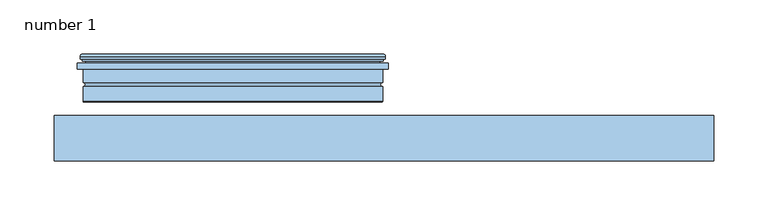
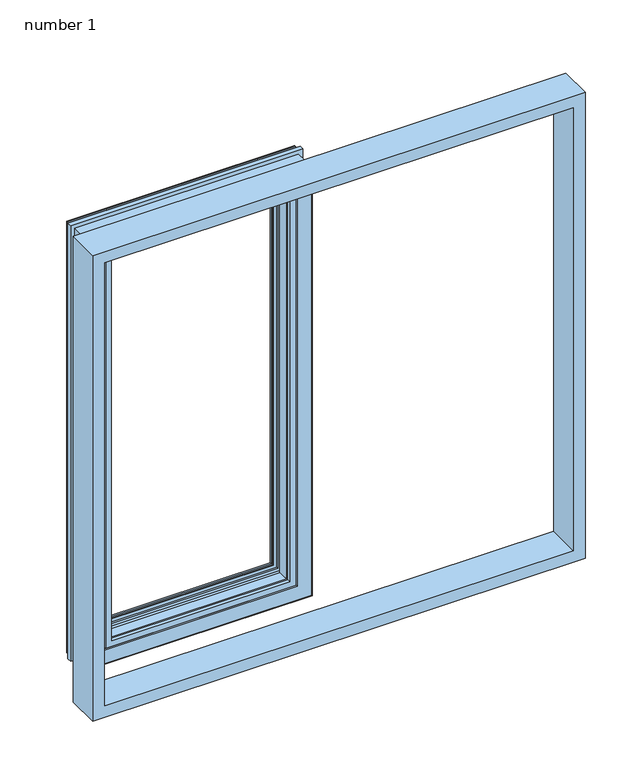
"""IFC4 building model written with IfcOpenShell, lengths in millimetres: window geometry, Window-Exterior-Sierra-Horizontal_Sliding_XO-36inch_Width-Standard : number 1."""

from ifc_helpers import new_model, si_unit, frame, origin, place, context, project, spatial, polyline, ellipse_curve, outline, extrude, source, transform, mapped, element, save
from ifc_brep_helpers import plane_surface, cylinder_surface, revolved_surface, advanced_brep


def number_1_632643b2(model_context):
    return source(origin(), model_context, "Body", "SolidModel", [
        advanced_brep(
        [(-250.12015, 35.099625, 967.49235), (-250.12015, 33.9637671, 967.49235), (-29.27985, 33.9637671, 967.49235), (-29.27985, 35.099625, 967.49235), (-248.2833265, 37.5426644, 969.3291735), (-248.0937762, 35.099625, 969.5187238), (-31.3062238, 35.099625, 969.5187238), (-31.1166735, 37.5426644, 969.3291735), (-256.08915, 40.078025, 961.52335), (-23.31085, 40.078025, 961.52335), (-256.08915, 42.465625, 961.52335), (-23.31085, 42.465625, 961.52335), (-280.77795, 40.078025, 936.83455), (-278.39035, 42.465625, 939.22215), (-1.00965, 42.465625, 939.22215), (1.37795, 40.078025, 936.83455), (-280.77795, 37.512625, 936.83455), (1.37795, 37.512625, 936.83455), (-278.74595, 35.836225, 938.86655), (-278.74595, 37.512625, 938.86655), (-0.65405, 37.512625, 938.86655), (-0.65405, 35.836225, 938.86655), (-275.44395, 33.931225, 942.16855), (-275.44395, 35.836225, 942.16855), (-3.95605, 35.836225, 942.16855), (-3.95605, 33.931225, 942.16855), (-283.36875, 28.317825, 934.24375), (-283.36875, 33.931225, 934.24375), (3.96875, 33.931225, 934.24375), (3.96875, 28.317825, 934.24375), (-278.06015, 16.125825, 939.55235), (-278.06015, 28.317825, 939.55235), (-1.33985, 28.317825, 939.55235), (-1.33985, 16.125825, 939.55235), (-278.06015, 12.163425, 939.55235), (-1.33985, 12.163425, 939.55235), (-278.06015, -1.171575, 939.55235), (-1.33985, -1.171575, 939.55235), (-277.24735, -1.984375, 940.36515), (-2.15265, -1.984375, 940.36515), (-258.95935, -0.103857, 958.65315), (-258.95935, -1.984375, 958.65315), (-20.44065, -1.984375, 958.65315), (-20.44065, -0.103857, 958.65315), (-257.3584612, -1.704057, 960.2540388), (-257.3584612, -0.103857, 960.2540388), (-22.0415388, -0.103857, 960.2540388), (-22.0415388, -1.704057, 960.2540388), (-249.8146612, 2.0638625, 967.7978388), (-249.8146612, -1.704057, 967.7978388), (-29.5853388, -1.704057, 967.7978388), (-29.5853388, 2.0638625, 967.7978388), (-246.6396612, 13.891543, 970.9728388), (-247.6523112, 2.0638625, 969.9601888), (-31.7476888, 2.0638625, 969.9601888), (-32.7603388, 13.891543, 970.9728388), (-258.95935, 11.5032541, 958.65315), (-256.5710612, 13.891543, 961.0414388), (-22.8289388, 13.891543, 961.0414388), (-20.44065, 11.5032541, 958.65315), (-258.95935, 32.940625, 958.65315), (-20.44065, 32.940625, 958.65315), (-254.3555891, 33.9637671, 963.2569109), (-255.3787312, 32.940625, 962.2337688), (-24.0212688, 32.940625, 962.2337688), (-25.0444109, 33.9637671, 963.2569109), (-29.27985, 33.9637671, 1470.90765), (-29.27985, 35.099625, 1470.90765), (-31.3062238, 35.099625, 1468.8812762), (-31.1166735, 37.5426644, 1469.0708265), (-23.31085, 40.078025, 1476.87665), (-23.31085, 42.465625, 1476.87665), (-1.00965, 42.465625, 1499.17785), (1.37795, 40.078025, 1501.56545), (1.37795, 37.512625, 1501.56545), (-0.65405, 37.512625, 1499.53345), (-0.65405, 35.836225, 1499.53345), (-3.95605, 35.836225, 1496.23145), (-3.95605, 33.931225, 1496.23145), (3.96875, 33.931225, 1504.15625), (3.96875, 28.317825, 1504.15625), (-1.33985, 28.317825, 1498.84765), (-1.33985, 16.125825, 1498.84765), (-1.33985, 12.163425, 1498.84765), (-1.33985, -1.171575, 1498.84765), (-2.15265, -1.984375, 1498.03485), (-20.44065, -1.984375, 1479.74685), (-20.44065, -0.103857, 1479.74685), (-22.0415388, -0.103857, 1478.1459612), (-22.0415388, -1.704057, 1478.1459612), (-29.5853388, -1.704057, 1470.6021612), (-29.5853388, 2.0638625, 1470.6021612), (-31.7476888, 2.0638625, 1468.4398112), (-32.7603388, 13.891543, 1467.4271612), (-22.8289388, 13.891543, 1477.3585612), (-20.44065, 11.5032541, 1479.74685), (-20.44065, 32.940625, 1479.74685), (-24.0212688, 32.940625, 1476.1662312), (-25.0444109, 33.9637671, 1475.1430891), (-250.12015, 33.9637671, 1470.90765), (-250.12015, 35.099625, 1470.90765), (-248.0937762, 35.099625, 1468.8812762), (-248.2833265, 37.5426644, 1469.0708265), (-256.08915, 40.078025, 1476.87665), (-256.08915, 42.465625, 1476.87665), (-278.39035, 42.465625, 1499.17785), (-280.77795, 40.078025, 1501.56545), (-280.77795, 37.512625, 1501.56545), (-278.74595, 37.512625, 1499.53345), (-278.74595, 35.836225, 1499.53345), (-275.44395, 35.836225, 1496.23145), (-275.44395, 33.931225, 1496.23145), (-283.36875, 33.931225, 1504.15625), (-283.36875, 28.317825, 1504.15625), (-278.06015, 28.317825, 1498.84765), (-278.06015, 16.125825, 1498.84765), (-278.06015, 12.163425, 1498.84765), (-278.06015, -1.171575, 1498.84765), (-277.24735, -1.984375, 1498.03485), (-258.95935, -1.984375, 1479.74685), (-258.95935, -0.103857, 1479.74685), (-257.3584612, -0.103857, 1478.1459612), (-257.3584612, -1.704057, 1478.1459612), (-249.8146612, -1.704057, 1470.6021612), (-249.8146612, 2.0638625, 1470.6021612), (-247.6523112, 2.0638625, 1468.4398112), (-246.6396612, 13.891543, 1467.4271612), (-256.5710612, 13.891543, 1477.3585612), (-258.95935, 11.5032541, 1479.74685), (-258.95935, 32.940625, 1479.74685), (-255.3787312, 32.940625, 1476.1662312), (-254.3555891, 33.9637671, 1475.1430891)],
        [
            (0, 1),
            (1, 2),
            (2, 3),
            (3, 0),
            (4, 5),
            (5, 6),
            (6, 7),
            (7, 4),
            (8, 4),
            (7, 9),
            (9, 8),
            (10, 8),
            (9, 11),
            (11, 10),
            (12, 13, ellipse_curve(frame((-278.39035, 40.078025, 939.22215), z_axis=(0.7071067811865475, 0.0, -0.7071067811865475), x_axis=(-0.7071067811865476, 0.0, -0.7071067811865474)), 3.3765763, 2.3876)),
            (13, 14),
            (14, 15, ellipse_curve(frame((-1.00965, 40.078025, 939.22215), z_axis=(-0.7071067811865475, 0.0, -0.7071067811865475), x_axis=(-0.7071067811865476, 0.0, 0.7071067811865474)), 3.3765763, 2.3876)),
            (15, 12),
            (16, 12),
            (15, 17),
            (17, 16),
            (18, 19),
            (19, 20),
            (20, 21),
            (21, 18),
            (22, 23),
            (23, 24),
            (24, 25),
            (25, 22),
            (26, 27),
            (27, 28),
            (28, 29),
            (29, 26),
            (30, 31),
            (31, 32),
            (32, 33),
            (33, 30),
            (34, 30, ellipse_curve(frame((-278.06015, 14.144625, 939.55235), z_axis=(-0.7071067811865475, 0.0, 0.7071067811865475), x_axis=(0.7071067811865476, 0.0, 0.7071067811865474)), 2.8018399, 1.9812)),
            (33, 35, ellipse_curve(frame((-1.33985, 14.144625, 939.55235), z_axis=(0.7071067811865475, 0.0, 0.7071067811865475), x_axis=(0.7071067811865476, 0.0, -0.7071067811865474)), 2.8018399, 1.9812)),
            (35, 34),
            (36, 34),
            (35, 37),
            (37, 36),
            (38, 36, ellipse_curve(frame((-277.24735, -1.171575, 940.36515), z_axis=(0.7071067811865475, 0.0, -0.7071067811865475), x_axis=(-0.7071067811865476, 0.0, -0.7071067811865474)), 1.1494728, 0.8128)),
            (37, 39, ellipse_curve(frame((-2.15265, -1.171575, 940.36515), z_axis=(-0.7071067811865475, 0.0, -0.7071067811865475), x_axis=(-0.7071067811865476, 0.0, 0.7071067811865474)), 1.1494728, 0.8128)),
            (39, 38),
            (40, 41),
            (41, 42),
            (42, 43),
            (43, 40),
            (44, 45),
            (45, 46),
            (46, 47),
            (47, 44),
            (48, 49),
            (49, 50),
            (50, 51),
            (51, 48),
            (52, 53),
            (53, 54),
            (54, 55),
            (55, 52),
            (56, 57),
            (57, 58),
            (58, 59),
            (59, 56),
            (60, 56),
            (59, 61),
            (61, 60),
            (62, 63),
            (63, 64),
            (64, 65),
            (65, 62),
            (2, 66),
            (66, 67),
            (67, 3),
            (6, 68),
            (68, 69),
            (69, 7),
            (69, 70),
            (70, 9),
            (70, 71),
            (71, 11),
            (14, 72),
            (72, 73, ellipse_curve(frame((-1.00965, 40.078025, 1499.17785), z_axis=(0.7071067811865475, 0.0, -0.7071067811865475), x_axis=(-0.7071067811865474, 0.0, -0.7071067811865476)), 3.3765763, 2.3876)),
            (73, 15),
            (73, 74),
            (74, 17),
            (20, 75),
            (75, 76),
            (76, 21),
            (24, 77),
            (77, 78),
            (78, 25),
            (28, 79),
            (79, 80),
            (80, 29),
            (32, 81),
            (81, 82),
            (82, 33),
            (82, 83, ellipse_curve(frame((-1.33985, 14.144625, 1498.84765), z_axis=(-0.7071067811865475, 0.0, 0.7071067811865475), x_axis=(0.7071067811865474, 0.0, 0.7071067811865476)), 2.8018399, 1.9812)),
            (83, 35),
            (83, 84),
            (84, 37),
            (84, 85, ellipse_curve(frame((-2.15265, -1.171575, 1498.03485), z_axis=(0.7071067811865475, 0.0, -0.7071067811865475), x_axis=(-0.7071067811865474, 0.0, -0.7071067811865476)), 1.1494728, 0.8128)),
            (85, 39),
            (42, 86),
            (86, 87),
            (87, 43),
            (46, 88),
            (88, 89),
            (89, 47),
            (50, 90),
            (90, 91),
            (91, 51),
            (54, 92),
            (92, 93),
            (93, 55),
            (58, 94),
            (94, 95),
            (95, 59),
            (95, 96),
            (96, 61),
            (64, 97),
            (97, 98),
            (98, 65),
            (66, 99),
            (99, 100),
            (100, 67),
            (68, 101),
            (101, 102),
            (102, 69),
            (102, 103),
            (103, 70),
            (103, 104),
            (104, 71),
            (72, 105),
            (105, 106, ellipse_curve(frame((-278.39035, 40.078025, 1499.17785), z_axis=(0.7071067811865475, 0.0, 0.7071067811865475), x_axis=(0.7071067811865476, 0.0, -0.7071067811865474)), 3.3765763, 2.3876)),
            (106, 73),
            (106, 107),
            (107, 74),
            (75, 108),
            (108, 109),
            (109, 76),
            (77, 110),
            (110, 111),
            (111, 78),
            (79, 112),
            (112, 113),
            (113, 80),
            (81, 114),
            (114, 115),
            (115, 82),
            (115, 116, ellipse_curve(frame((-278.06015, 14.144625, 1498.84765), z_axis=(-0.7071067811865475, 0.0, -0.7071067811865475), x_axis=(-0.7071067811865476, 0.0, 0.7071067811865474)), 2.8018399, 1.9812)),
            (116, 83),
            (116, 117),
            (117, 84),
            (117, 118, ellipse_curve(frame((-277.24735, -1.171575, 1498.03485), z_axis=(0.7071067811865475, 0.0, 0.7071067811865475), x_axis=(0.7071067811865476, 0.0, -0.7071067811865474)), 1.1494728, 0.8128)),
            (118, 85),
            (86, 119),
            (119, 120),
            (120, 87),
            (88, 121),
            (121, 122),
            (122, 89),
            (90, 123),
            (123, 124),
            (124, 91),
            (92, 125),
            (125, 126),
            (126, 93),
            (94, 127),
            (127, 128),
            (128, 95),
            (128, 129),
            (129, 96),
            (97, 130),
            (130, 131),
            (131, 98),
            (131, 62),
            (1, 99),
            (0, 100),
            (5, 101),
            (4, 102),
            (8, 103),
            (10, 104),
            (13, 105),
            (12, 106),
            (16, 107),
            (19, 108),
            (18, 109),
            (23, 110),
            (22, 111),
            (27, 112),
            (26, 113),
            (31, 114),
            (30, 115),
            (34, 116),
            (36, 117),
            (38, 118),
            (41, 119),
            (40, 120),
            (45, 121),
            (44, 122),
            (49, 123),
            (48, 124),
            (53, 125),
            (52, 126),
            (57, 127),
            (56, 128),
            (60, 129),
            (63, 130),
        ],
        [
            plane_surface(frame((-250.12015, 33.9637671, 967.49235), z_axis=(0.0, 0.0, 1.0), x_axis=(1.0, 0.0, 0.0))),
            plane_surface(frame((-248.0937762, 35.099625, 969.5187238), z_axis=(0.0, 0.07735544009934271, 0.9970035786731345), x_axis=(1.0, 0.0, 0.0))),
            plane_surface(frame((-248.2833265, 37.5426644, 969.3291735), z_axis=(0.0, 0.9510889261909004, 0.3089172291683326), x_axis=(1.0, 0.0, 0.0))),
            plane_surface(frame((-256.08915, 40.078025, 961.52335), z_axis=(0.0, 0.0, 1.0), x_axis=(1.0, 0.0, 0.0))),
            cylinder_surface(frame((-283.36875, 40.078025, 939.22215), z_axis=(-1.0, 0.0, 0.0), x_axis=(0.0, -1.0, 0.0)), 2.3876),
            plane_surface(frame((-280.77795, 40.078025, 936.83455), z_axis=(0.0, 0.0, -1.0), x_axis=(1.0, 0.0, 0.0))),
            plane_surface(frame((-278.74595, 37.512625, 938.86655), z_axis=(0.0, 0.0, -1.0), x_axis=(1.0, 0.0, 0.0))),
            plane_surface(frame((-275.44395, 35.836225, 942.16855), z_axis=(0.0, 0.0, -1.0), x_axis=(1.0, 0.0, 0.0))),
            plane_surface(frame((-283.36875, 33.931225, 934.24375), z_axis=(0.0, 0.0, -1.0), x_axis=(1.0, 0.0, 0.0))),
            plane_surface(frame((-278.06015, 28.317825, 939.55235), z_axis=(0.0, 0.0, -1.0), x_axis=(1.0, 0.0, 0.0))),
            revolved_surface(polyline([(0.6413499930890225, 12.163425, 939.55235), (-280.04134999308906, 12.163425, 939.55235)]), (-283.36875, 14.144625, 939.55235), (1.0, 0.0, 0.0)),
            plane_surface(frame((-278.06015, 12.163425, 939.55235), z_axis=(0.0, 0.0, -1.0), x_axis=(1.0, 0.0, 0.0))),
            cylinder_surface(frame((-283.36875, -1.171575, 940.36515), z_axis=(-1.0, 0.0, 0.0), x_axis=(0.0, -1.0, 0.0)), 0.8128),
            plane_surface(frame((-258.95935, -1.984375, 958.65315), z_axis=(0.0, 0.0, 1.0), x_axis=(1.0, 0.0, 0.0))),
            plane_surface(frame((-257.3584612, -0.103857, 960.2540388), z_axis=(0.0, 0.0, -1.0), x_axis=(1.0, 0.0, 0.0))),
            plane_surface(frame((-249.8146612, -1.704057, 967.7978388), z_axis=(0.0, 0.0, 1.0), x_axis=(1.0, 0.0, 0.0))),
            plane_surface(frame((-247.6523112, 2.0638625, 969.9601888), z_axis=(0.0, -0.08530487454184647, 0.996354895797376), x_axis=(1.0, 0.0, 0.0))),
            plane_surface(frame((-256.5710612, 13.891543, 961.0414388), z_axis=(0.0, 0.7071067811865713, -0.7071067811865238), x_axis=(1.0, 0.0, 0.0))),
            plane_surface(frame((-258.95935, 11.5032541, 958.65315), z_axis=(0.0, 0.0, 1.0), x_axis=(1.0, 0.0, 0.0))),
            plane_surface(frame((-255.3787312, 32.940625, 962.2337688), z_axis=(0.0, -0.7071067811861558, 0.7071067811869393), x_axis=(1.0, 0.0, 0.0))),
            plane_surface(frame((-29.27985, 33.9637671, 967.49235), z_axis=(-1.0, 0.0, 0.0), x_axis=(0.0, 0.0, 1.0))),
            plane_surface(frame((-31.3062238, 35.099625, 969.5187238), z_axis=(-0.9970035786731345, 0.07735544009934266, 0.0), x_axis=(0.0, 0.0, 1.0))),
            plane_surface(frame((-31.1166735, 37.5426644, 969.3291735), z_axis=(-0.30891722916833264, 0.9510889261909004, 0.0), x_axis=(0.0, 0.0, 1.0))),
            plane_surface(frame((-23.31085, 40.078025, 961.52335), z_axis=(-1.0, 0.0, 0.0), x_axis=(0.0, 0.0, 1.0))),
            cylinder_surface(frame((-1.00965, 40.078025, 934.24375), z_axis=(0.0, 0.0, -1.0), x_axis=(0.0, -1.0, 0.0)), 2.3876),
            plane_surface(frame((1.37795, 40.078025, 936.83455), z_axis=(1.0, 0.0, 0.0), x_axis=(0.0, 0.0, 1.0))),
            plane_surface(frame((-0.65405, 37.512625, 938.86655), z_axis=(1.0, 0.0, 0.0), x_axis=(0.0, 0.0, 1.0))),
            plane_surface(frame((-3.95605, 35.836225, 942.16855), z_axis=(1.0, 0.0, 0.0), x_axis=(0.0, 0.0, 1.0))),
            plane_surface(frame((3.96875, 33.931225, 934.24375), z_axis=(1.0, 0.0, 0.0), x_axis=(0.0, 0.0, 1.0))),
            plane_surface(frame((-1.33985, 28.317825, 939.55235), z_axis=(1.0, 0.0, 0.0), x_axis=(0.0, 0.0, 1.0))),
            revolved_surface(polyline([(-1.33985, 12.163425, 1500.828849993089), (-1.33985, 12.163425, 937.571150006911)]), (-1.33985, 14.144625, 934.24375), (0.0, 0.0, 1.0)),
            plane_surface(frame((-1.33985, 12.163425, 939.55235), z_axis=(1.0, 0.0, 0.0), x_axis=(0.0, 0.0, 1.0))),
            cylinder_surface(frame((-2.15265, -1.171575, 934.24375), z_axis=(0.0, 0.0, -1.0), x_axis=(0.0, -1.0, 0.0)), 0.8128),
            plane_surface(frame((-20.44065, -1.984375, 958.65315), z_axis=(-1.0, 0.0, 0.0), x_axis=(0.0, 0.0, 1.0))),
            plane_surface(frame((-22.0415388, -0.103857, 960.2540388), z_axis=(1.0, 0.0, 0.0), x_axis=(0.0, 0.0, 1.0))),
            plane_surface(frame((-29.5853388, -1.704057, 967.7978388), z_axis=(-1.0, 0.0, 0.0), x_axis=(0.0, 0.0, 1.0))),
            plane_surface(frame((-31.7476888, 2.0638625, 969.9601888), z_axis=(-0.996354895797376, -0.08530487454184653, 0.0), x_axis=(0.0, 0.0, 1.0))),
            plane_surface(frame((-22.8289388, 13.891543, 961.0414388), z_axis=(0.7071067811865238, 0.7071067811865713, 0.0), x_axis=(0.0, 0.0, 1.0))),
            plane_surface(frame((-20.44065, 11.5032541, 958.65315), z_axis=(-1.0, 0.0, 0.0), x_axis=(0.0, 0.0, 1.0))),
            plane_surface(frame((-24.0212688, 32.940625, 962.2337688), z_axis=(-0.7071067811869393, -0.7071067811861558, 0.0), x_axis=(0.0, 0.0, 1.0))),
            plane_surface(frame((-29.27985, 33.9637671, 1470.90765), z_axis=(0.0, 0.0, -1.0), x_axis=(-1.0, 0.0, 0.0))),
            plane_surface(frame((-31.3062238, 35.099625, 1468.8812762), z_axis=(0.0, 0.0773554400993426, -0.9970035786731345), x_axis=(-1.0, 0.0, 0.0))),
            plane_surface(frame((-31.1166735, 37.5426644, 1469.0708265), z_axis=(0.0, 0.9510889261909004, -0.3089172291683327), x_axis=(-1.0, 0.0, 0.0))),
            plane_surface(frame((-23.31085, 40.078025, 1476.87665), z_axis=(0.0, 0.0, -1.0), x_axis=(-1.0, 0.0, 0.0))),
            cylinder_surface(frame((3.96875, 40.078025, 1499.17785), z_axis=(1.0, 0.0, 0.0), x_axis=(0.0, -1.0, 0.0)), 2.3876),
            plane_surface(frame((1.37795, 40.078025, 1501.56545), z_axis=(0.0, 0.0, 1.0), x_axis=(-1.0, 0.0, 0.0))),
            plane_surface(frame((-0.65405, 37.512625, 1499.53345), z_axis=(0.0, 0.0, 1.0), x_axis=(-1.0, 0.0, 0.0))),
            plane_surface(frame((-3.95605, 35.836225, 1496.23145), z_axis=(0.0, 0.0, 1.0), x_axis=(-1.0, 0.0, 0.0))),
            plane_surface(frame((3.96875, 33.931225, 1504.15625), z_axis=(0.0, 0.0, 1.0), x_axis=(-1.0, 0.0, 0.0))),
            plane_surface(frame((-1.33985, 28.317825, 1498.84765), z_axis=(0.0, 0.0, 1.0), x_axis=(-1.0, 0.0, 0.0))),
            revolved_surface(polyline([(-280.04134999308906, 12.163425, 1498.84765), (0.6413499930890376, 12.163425, 1498.84765)]), (3.96875, 14.144625, 1498.84765), (-1.0, 0.0, 0.0)),
            plane_surface(frame((-1.33985, 12.163425, 1498.84765), z_axis=(0.0, 0.0, 1.0), x_axis=(-1.0, 0.0, 0.0))),
            cylinder_surface(frame((3.96875, -1.171575, 1498.03485), z_axis=(1.0, 0.0, 0.0), x_axis=(0.0, -1.0, 0.0)), 0.8128),
            plane_surface(frame((-20.44065, -1.984375, 1479.74685), z_axis=(0.0, 0.0, -1.0), x_axis=(-1.0, 0.0, 0.0))),
            plane_surface(frame((-22.0415388, -0.103857, 1478.1459612), z_axis=(0.0, 0.0, 1.0), x_axis=(-1.0, 0.0, 0.0))),
            plane_surface(frame((-29.5853388, -1.704057, 1470.6021612), z_axis=(0.0, 0.0, -1.0), x_axis=(-1.0, 0.0, 0.0))),
            plane_surface(frame((-31.7476888, 2.0638625, 1468.4398112), z_axis=(0.0, -0.08530487454184658, -0.996354895797376), x_axis=(-1.0, 0.0, 0.0))),
            plane_surface(frame((-22.8289388, 13.891543, 1477.3585612), z_axis=(0.0, 0.7071067811865713, 0.7071067811865238), x_axis=(-1.0, 0.0, 0.0))),
            plane_surface(frame((-20.44065, 11.5032541, 1479.74685), z_axis=(0.0, 0.0, -1.0), x_axis=(-1.0, 0.0, 0.0))),
            plane_surface(frame((-24.0212688, 32.940625, 1476.1662312), z_axis=(0.0, -0.7071067811861558, -0.7071067811869393), x_axis=(-1.0, 0.0, 0.0))),
            plane_surface(frame((-254.3555891, 33.9637671, 1475.1430891), z_axis=(0.0, -1.0, 0.0), x_axis=(0.0, 0.0, -1.0))),
            plane_surface(frame((-250.12015, 33.9637671, 1470.90765), z_axis=(1.0, 0.0, 0.0), x_axis=(0.0, 0.0, -1.0))),
            plane_surface(frame((-250.12015, 35.099625, 1470.90765), z_axis=(0.0, -1.0, 0.0), x_axis=(0.0, 0.0, -1.0))),
            plane_surface(frame((-248.0937762, 35.099625, 1468.8812762), z_axis=(0.9970035786731345, 0.07735544009934266, 0.0), x_axis=(0.0, 0.0, -1.0))),
            plane_surface(frame((-248.2833265, 37.5426644, 1469.0708265), z_axis=(0.30891722916833264, 0.9510889261909004, 0.0), x_axis=(0.0, 0.0, -1.0))),
            plane_surface(frame((-256.08915, 40.078025, 1476.87665), z_axis=(1.0, 0.0, 0.0), x_axis=(0.0, 0.0, -1.0))),
            plane_surface(frame((-256.08915, 42.465625, 1476.87665), z_axis=(0.0, 1.0, 0.0), x_axis=(0.0, 0.0, -1.0))),
            cylinder_surface(frame((-278.39035, 40.078025, 1504.15625), z_axis=(0.0, 0.0, 1.0), x_axis=(0.0, -1.0, 0.0)), 2.3876),
            plane_surface(frame((-280.77795, 40.078025, 1501.56545), z_axis=(-1.0, 0.0, 0.0), x_axis=(0.0, 0.0, -1.0))),
            plane_surface(frame((-280.77795, 37.512625, 1501.56545), z_axis=(0.0, -1.0, 0.0), x_axis=(0.0, 0.0, -1.0))),
            plane_surface(frame((-278.74595, 37.512625, 1499.53345), z_axis=(-1.0, 0.0, 0.0), x_axis=(0.0, 0.0, -1.0))),
            plane_surface(frame((-278.74595, 35.836225, 1499.53345), z_axis=(0.0, -1.0, 0.0), x_axis=(0.0, 0.0, -1.0))),
            plane_surface(frame((-275.44395, 35.836225, 1496.23145), z_axis=(-1.0, 0.0, 0.0), x_axis=(0.0, 0.0, -1.0))),
            plane_surface(frame((-275.44395, 33.931225, 1496.23145), z_axis=(0.0, 1.0, 0.0), x_axis=(0.0, 0.0, -1.0))),
            plane_surface(frame((-283.36875, 33.931225, 1504.15625), z_axis=(-1.0, 0.0, 0.0), x_axis=(0.0, 0.0, -1.0))),
            plane_surface(frame((-283.36875, 28.317825, 1504.15625), z_axis=(0.0, -1.0, 0.0), x_axis=(0.0, 0.0, -1.0))),
            plane_surface(frame((-278.06015, 28.317825, 1498.84765), z_axis=(-1.0, 0.0, 0.0), x_axis=(0.0, 0.0, -1.0))),
            revolved_surface(polyline([(-278.06015, 12.163425, 937.571150006911), (-278.06015, 12.163425, 1500.828849993089)]), (-278.06015, 14.144625, 1504.15625), (0.0, 0.0, -1.0)),
            plane_surface(frame((-278.06015, 12.163425, 1498.84765), z_axis=(-1.0, 0.0, 0.0), x_axis=(0.0, 0.0, -1.0))),
            cylinder_surface(frame((-277.24735, -1.171575, 1504.15625), z_axis=(0.0, 0.0, 1.0), x_axis=(0.0, -1.0, 0.0)), 0.8128),
            plane_surface(frame((-277.24735, -1.984375, 1498.03485), z_axis=(0.0, -1.0, 0.0), x_axis=(0.0, 0.0, -1.0))),
            plane_surface(frame((-258.95935, -1.984375, 1479.74685), z_axis=(1.0, 0.0, 0.0), x_axis=(0.0, 0.0, -1.0))),
            plane_surface(frame((-258.95935, -0.103857, 1479.74685), z_axis=(0.0, -1.0, 0.0), x_axis=(0.0, 0.0, -1.0))),
            plane_surface(frame((-257.3584612, -0.103857, 1478.1459612), z_axis=(-1.0, 0.0, 0.0), x_axis=(0.0, 0.0, -1.0))),
            plane_surface(frame((-257.3584612, -1.704057, 1478.1459612), z_axis=(0.0, -1.0, 0.0), x_axis=(0.0, 0.0, -1.0))),
            plane_surface(frame((-249.8146612, -1.704057, 1470.6021612), z_axis=(1.0, 0.0, 0.0), x_axis=(0.0, 0.0, -1.0))),
            plane_surface(frame((-249.8146612, 2.0638625, 1470.6021612), z_axis=(0.0, -1.0, 0.0), x_axis=(0.0, 0.0, -1.0))),
            plane_surface(frame((-247.6523112, 2.0638625, 1468.4398112), z_axis=(0.996354895797376, -0.08530487454184653, 0.0), x_axis=(0.0, 0.0, -1.0))),
            plane_surface(frame((-246.6396612, 13.891543, 1467.4271612), z_axis=(0.0, 1.0, 0.0), x_axis=(0.0, 0.0, -1.0))),
            plane_surface(frame((-256.5710612, 13.891543, 1477.3585612), z_axis=(-0.7071067811865238, 0.7071067811865713, 0.0), x_axis=(0.0, 0.0, -1.0))),
            plane_surface(frame((-258.95935, 11.5032541, 1479.74685), z_axis=(1.0, 0.0, 0.0), x_axis=(0.0, 0.0, -1.0))),
            plane_surface(frame((-258.95935, 32.940625, 1479.74685), z_axis=(0.0, -1.0, 0.0), x_axis=(0.0, 0.0, -1.0))),
            plane_surface(frame((-255.3787312, 32.940625, 1476.1662312), z_axis=(0.7071067811869393, -0.7071067811861558, 0.0), x_axis=(0.0, 0.0, -1.0))),
        ],
        [
            (0, [[1, 2, 3, 4]]),
            (1, [[5, 6, 7, 8]]),
            (2, [[9, -8, 10, 11]]),
            (3, [[12, -11, 13, 14]]),
            (4, [[15, 16, 17, 18]]),
            (5, [[19, -18, 20, 21]]),
            (6, [[22, 23, 24, 25]]),
            (7, [[26, 27, 28, 29]]),
            (8, [[30, 31, 32, 33]]),
            (9, [[34, 35, 36, 37]]),
            (10, [[38, -37, 39, 40]]),
            (11, [[41, -40, 42, 43]]),
            (12, [[44, -43, 45, 46]]),
            (13, [[47, 48, 49, 50]]),
            (14, [[51, 52, 53, 54]]),
            (15, [[55, 56, 57, 58]]),
            (16, [[59, 60, 61, 62]]),
            (17, [[63, 64, 65, 66]]),
            (18, [[67, -66, 68, 69]]),
            (19, [[70, 71, 72, 73]]),
            (20, [[-3, 74, 75, 76]]),
            (21, [[-7, 77, 78, 79]]),
            (22, [[-10, -79, 80, 81]]),
            (23, [[-13, -81, 82, 83]]),
            (24, [[-17, 84, 85, 86]]),
            (25, [[-20, -86, 87, 88]]),
            (26, [[-24, 89, 90, 91]]),
            (27, [[-28, 92, 93, 94]]),
            (28, [[-32, 95, 96, 97]]),
            (29, [[-36, 98, 99, 100]]),
            (30, [[-39, -100, 101, 102]]),
            (31, [[-42, -102, 103, 104]]),
            (32, [[-45, -104, 105, 106]]),
            (33, [[-49, 107, 108, 109]]),
            (34, [[-53, 110, 111, 112]]),
            (35, [[-57, 113, 114, 115]]),
            (36, [[-61, 116, 117, 118]]),
            (37, [[-65, 119, 120, 121]]),
            (38, [[-68, -121, 122, 123]]),
            (39, [[-72, 124, 125, 126]]),
            (40, [[-75, 127, 128, 129]]),
            (41, [[-78, 130, 131, 132]]),
            (42, [[-80, -132, 133, 134]]),
            (43, [[-82, -134, 135, 136]]),
            (44, [[-85, 137, 138, 139]]),
            (45, [[-87, -139, 140, 141]]),
            (46, [[-90, 142, 143, 144]]),
            (47, [[-93, 145, 146, 147]]),
            (48, [[-96, 148, 149, 150]]),
            (49, [[-99, 151, 152, 153]]),
            (50, [[-101, -153, 154, 155]]),
            (51, [[-103, -155, 156, 157]]),
            (52, [[-105, -157, 158, 159]]),
            (53, [[-108, 160, 161, 162]]),
            (54, [[-111, 163, 164, 165]]),
            (55, [[-114, 166, 167, 168]]),
            (56, [[-117, 169, 170, 171]]),
            (57, [[-120, 172, 173, 174]]),
            (58, [[-122, -174, 175, 176]]),
            (59, [[-125, 177, 178, 179]]),
            (60, [[-126, -179, 180, -73], [181, -127, -74, -2]]),
            (61, [[-128, -181, -1, 182]]),
            (62, [[-76, -129, -182, -4], [183, -130, -77, -6]]),
            (63, [[-131, -183, -5, 184]]),
            (64, [[-133, -184, -9, 185]]),
            (65, [[-135, -185, -12, 186]]),
            (66, [[187, -137, -84, -16], [-83, -136, -186, -14]]),
            (67, [[-138, -187, -15, 188]]),
            (68, [[-140, -188, -19, 189]]),
            (69, [[-88, -141, -189, -21], [190, -142, -89, -23]]),
            (70, [[-143, -190, -22, 191]]),
            (71, [[-91, -144, -191, -25], [192, -145, -92, -27]]),
            (72, [[-146, -192, -26, 193]]),
            (73, [[194, -148, -95, -31], [-94, -147, -193, -29]]),
            (74, [[-149, -194, -30, 195]]),
            (75, [[-97, -150, -195, -33], [196, -151, -98, -35]]),
            (76, [[-152, -196, -34, 197]]),
            (77, [[-154, -197, -38, 198]]),
            (78, [[-156, -198, -41, 199]]),
            (79, [[-158, -199, -44, 200]]),
            (80, [[-106, -159, -200, -46], [201, -160, -107, -48]]),
            (81, [[-161, -201, -47, 202]]),
            (82, [[-109, -162, -202, -50], [203, -163, -110, -52]]),
            (83, [[-164, -203, -51, 204]]),
            (84, [[-112, -165, -204, -54], [205, -166, -113, -56]]),
            (85, [[-167, -205, -55, 206]]),
            (86, [[-115, -168, -206, -58], [207, -169, -116, -60]]),
            (87, [[-170, -207, -59, 208]]),
            (88, [[209, -172, -119, -64], [-118, -171, -208, -62]]),
            (89, [[-173, -209, -63, 210]]),
            (90, [[-175, -210, -67, 211]]),
            (91, [[-123, -176, -211, -69], [212, -177, -124, -71]]),
            (92, [[-178, -212, -70, -180]]),
        ],
    ),
        extrude(outline(polyline([(1524.0, 304.8), (1524.0, -304.8), (914.4, -304.8), (914.4, 304.8), (1524.0, 304.8)]), holes=[polyline([(929.4367932, 289.7632068), (929.4367932, -289.7632068), (1508.9632068, -289.7632068), (1508.9632068, 289.7632068), (929.4367932, 289.7632068)])]), frame((0.0, -56.35625, 0.0), z_axis=(0.0, 1.0, 0.0), x_axis=(0.0, 0.0, 1.0)), (0.0, 0.0, 1.0), 41.7512996),
    ])


if __name__ == "__main__":
    model = new_model("IFC4")
    model_context = context("Model", 3, world=origin())
    ifc_project = project(units=[si_unit("LENGTHUNIT", "METRE", prefix="MILLI")], contexts=[model_context])
    site = spatial("IfcSite", under=ifc_project)
    building = spatial("IfcBuilding", under=site)
    placement = place(None, origin())
    number_1_shape = number_1_632643b2(model_context)
    element("IfcWindow", 1, ObjectType="Window-Exterior-Sierra-Horizontal_Sliding_XO-36inch_Width-Standard : number 1", at=placement, inside=building, context=model_context, shape_type="MappedRepresentation", body=[
        mapped(number_1_shape, transform((0.0, 0.0, 0.0), x_axis=(1.0, 0.0, 0.0), y_axis=(0.0, 1.0, 0.0), z_axis=(0.0, 0.0, 1.0))),
    ])
    save(model, "model.ifc")

# Revit data of these elements
# Type "Window-Exterior-Sierra-Horizontal_Sliding_XO-36inch_Width-Standard : number 1"
#   Type Mark = "55"
#   URL = "http://www.sierrapacificwindows.com"
#   Triple Glaze Note = "Triple glazed options with respective limits"
#   Simulite Note = "Custom Simulite Options Available"
#   Product data url = "https://bimobject.com/sierrapacificwindows/product/sierrapacificwindows_horizontal-sliding-windows"
#   Product Page URL = "http://www.sierrapacificwindows.com/horizontal-sliding-windows.cfm"
#   Product Documentation Link = "http://www.sierrapacificwindows.com/architectural/drawings/pdfs/c-ws_13.pdf"
#   Model = "C-WS-3648"
#   Manufacturer = "Sierra Pacific Windows"
#   Jamb Extension Note = "Extension Jamb may be applied on some applications. Contact your SPW sales rep. for more information"
#   Glass Type = "Insulated Glass"
#   Description = "Energy efficient, durable, and secure window"
#   Construction Type = "Wood/Clad"
#   Assembly Code = "B2030230"
#   Window Pane Thickness = 0' - 0 3/4"
#   Vertical Simulite Length = 1' - 9"
#   Thickness = 0' - 1 3/4"
#   Simulite Wood Thickness Vertical = 0' - 0 11/32"
#   Simulite Wood Thickness Horizontal = 0' - 0 13/32"
#   Simulite Width = 0' - 0 7/8"
#   Simulite Clad Thickness Vertical = 0' - 0 11/32"
#   Simulite Clad Thickness Horizontal = 0' - 0 13/32"
#   Setback = 0' - 0"
#   Rough Width = 2' - 0 3/4"
#   Rough Height = 1' - 8 3/4"
#   Quarter Window Width = 0' - 6 1/2"
#   Interior Setback = 0' - 0"
#   Horizontal Simulite Length = 0' - 9 1/8"
#   Half Frame Width = 1' - 0 7/8"
#   Frame Width = 2' - 0"
#   Height = 1' - 8"
#   Width = 2' - 0"
#   Frame Height = 1' - 8"
#   First Simulite Width = 0' - 8 7/16"
#   First Simulite Height = 1' - 7 9/16"
#   Default Sill Height = 3' - 0"
#   Actual Width = 2' - 0"
#   Actual Height = 2' - 0"
#   Actual Half Width = 1' - 0"
#   Actual Glass Width = 0' - 8 7/16"
#   Actual Glass Height = 1' - 7 9/16"
#   Total Number of Lites Per Panel = 1
#   Simulites Visibility = yes
#   Number of Vertical Simulites Greater than One = 2
#   Number of Vertical Lites Per Panel = 1
#   Number of Horizontal Simulites Greater than One = 2
#   Number of Horizontal Lites Per Panel = 1
#   Vertical Simulite Type = element 483283
#   Interior Simulite = Wood - Sierra Pacific - Pine
#   Interior Panel Material = Wood - Sierra Pacific - Pine
#   Horizontal Simulite Type = element 483288
#   Glass = Glass - Sierra Doors - Clear
#   Frame = Paint - Sierra Pacific - White 001
#   Exterior Simulite = Paint - Sierra Pacific - White 001
#   Exterior Panel Material = Paint - Sierra Pacific - White 001
#   Wall Closure = (empty or 0)
# Element 1 (IfcWindow, "Window-Exterior-Sierra-Horizontal_Sliding_XO-36inch_Width-Standard : number 1")
#   Materials on its faces: "Wood - Sierra Pacific - Pine", "Paint - Sierra Pacific - White 001", "Glass - Sierra Doors - Clear"
# Materials
#   "Wood - Sierra Pacific - Pine": class "Miscellaneous", colour RGB 136 105 68, transparency 0
#   "Glass - Sierra Doors - Clear": class "Glass", colour RGB 0 0 255, transparency 0.75
#   "Paint - Sierra Pacific - White 001": class "Miscellaneous", colour RGB 111 112 111, transparency 0
